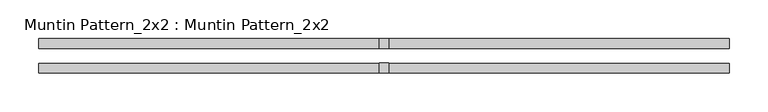
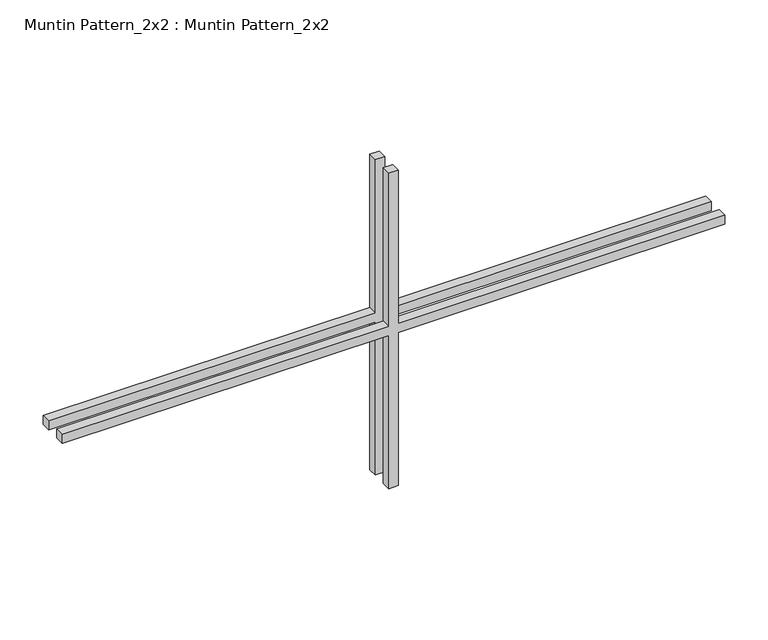
"""IFC4 building model written with IfcOpenShell, lengths in millimetres: proxy geometry, Muntin Pattern_2x2 : Muntin Pattern_2x2."""

from ifc_helpers import new_model, si_unit, frame, origin, place, context, project, spatial, polyline, outline, extrude, source, transform, mapped, element, save


def muntin_pattern_2x2_muntin_pattern_2x2_af2132b9(model_context):
    return source(origin(), model_context, "Body", "SweptSolid", [
        extrude(outline(polyline([(230.1875, -6.35), (230.1875, -444.5), (217.4875, -444.5), (217.4875, -6.35), (0.0, -6.35), (0.0, 6.35), (217.4875, 6.35), (217.4875, 444.5), (230.1875, 444.5), (230.1875, 6.35), (447.675, 6.35), (447.675, -6.35), (230.1875, -6.35)])), frame((0.0, 9.525, 0.0), z_axis=(0.0, 1.0, 0.0), x_axis=(0.0, 0.0, 1.0)), (0.0, 0.0, 1.0), 12.7),
        extrude(outline(polyline([(230.1875, -6.35), (230.1875, -444.5), (217.4875, -444.5), (217.4875, -6.35), (0.0, -6.35), (0.0, 6.35), (217.4875, 6.35), (217.4875, 444.5), (230.1875, 444.5), (230.1875, 6.35), (447.675, 6.35), (447.675, -6.35), (230.1875, -6.35)])), frame((0.0, -22.225, 0.0), z_axis=(0.0, 1.0, 0.0), x_axis=(0.0, 0.0, 1.0)), (0.0, 0.0, 1.0), 12.7),
    ])


if __name__ == "__main__":
    model = new_model("IFC4")
    model_context = context("Model", 3, world=origin())
    ifc_project = project(units=[si_unit("LENGTHUNIT", "METRE", prefix="MILLI")], contexts=[model_context])
    site = spatial("IfcSite", under=ifc_project)
    building = spatial("IfcBuilding", under=site)
    placement = place(None, origin())
    muntin_pattern_2x2_muntin_pattern_2x2_shape = muntin_pattern_2x2_muntin_pattern_2x2_af2132b9(model_context)
    element("IfcBuildingElementProxy", 1, Name="Muntin Pattern_2x2 : Muntin Pattern_2x2", ObjectType="Muntin Pattern_2x2 : Muntin Pattern_2x2", at=placement, inside=building, context=model_context, shape_type="MappedRepresentation", body=[
        mapped(muntin_pattern_2x2_muntin_pattern_2x2_shape, transform((0.0, 0.0, 0.0), x_axis=(1.0, 0.0, 0.0), y_axis=(0.0, 1.0, 0.0), z_axis=(0.0, 0.0, 1.0))),
    ])
    save(model, "model.ifc")

# Revit data of these elements
# Type "Muntin Pattern_2x2 : Muntin Pattern_2x2"
#   Width [instance default] = 4' - 0"
#   Thickness = 0' - 0 1/2"
#   Height [instance default] = 4' - 0"
#   Distance = 0' - 0 3/4"
#   Interior Material [instance default] = none
#   Exterior Material [instance default] = none
# Element 1 (IfcBuildingElementProxy, "Muntin Pattern_2x2 : Muntin Pattern_2x2")
#   Width = 2' - 11"
#   Height = 1' - 5 5/8"
#   Interior Material = Wood - Stained
#   Exterior Material = Clad - White
#   Materials on its faces: "Clad - White", "Wood - Stained"
# Materials
#   "Clad - White": class "Wood", colour RGB 242 242 238, transparency 0, Cost = 0
#   "Wood - Stained": class "Wood", colour RGB 224 178 126, transparency 0, Cost = 0
